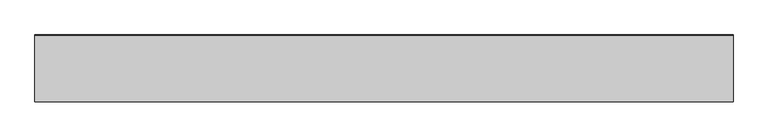
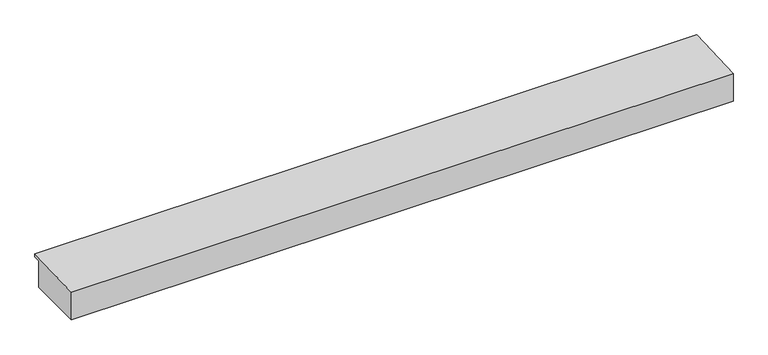
"""IFC4 building model written with IfcOpenShell, lengths in millimetres: proxy geometry, Generic Models 7:Generic Models 1:2:Generic Models 1:2 : Generic Models 7:Generic Models 1:337419:12 : Generic Models 7:Generic Models 1:2:Generic Models 1:2 : Generic Models 7:Generic Models 1:337419:306751."""

from ifc_helpers import new_model, si_unit, frame, origin, place, context, project, spatial, polyline, outline, extrude, source, transform, mapped, element, save


def generic_models_a1c6fa57(model_context):
    return source(origin(), model_context, "Body", "SweptSolid", [
        extrude(outline(polyline([(-578769.8021, 3730.7203868), (-578769.3002989, 3718.0302757), (-578794.3163841, 3716.9879388), (-578794.3163841, 3614.6261997), (-579001.9953617, 3614.6261997), (-579001.9953617, 3721.0456676), (-578769.8021, 3730.7203868)])), frame((591306.0367239, 0.0, 0.0), z_axis=(1.0, 0.0, 0.0), x_axis=(0.0, 1.0, 0.0)), (0.0, 0.0, 1.0), 2432.05),
    ])


if __name__ == "__main__":
    model = new_model("IFC4")
    model_context = context("Model", 3, world=origin())
    ifc_project = project(units=[si_unit("LENGTHUNIT", "METRE", prefix="MILLI")], contexts=[model_context])
    site = spatial("IfcSite", under=ifc_project)
    building = spatial("IfcBuilding", under=site)
    placement = place(None, origin())
    generic_models_shape = generic_models_a1c6fa57(model_context)
    element("IfcBuildingElementProxy", 1, Name="Generic Models 7:Generic Models 1:2:Generic Models 1:2 : Generic Models 7:Generic Models 1:337419:12 : Generic Models 7:Generic Models 1:2:Generic Models 1:2 : Generic Models 7:Generic Models 1:337419:306751", ObjectType="Generic Models 7:Generic Models 1:2:Generic Models 1:2 : Generic Models 7:Generic Models 1:337419:12 : Generic Models 7:Generic Models 1:2:Generic Models 1:2 : Generic Models 7:Generic Models 1:337419:306751", at=placement, inside=building, context=model_context, shape_type="MappedRepresentation", body=[
        mapped(generic_models_shape, transform((0.0, 0.0, 0.0), x_axis=(1.0, 0.0, 0.0), y_axis=(0.0, 1.0, 0.0), z_axis=(0.0, 0.0, 1.0))),
    ])
    save(model, "model.ifc")

# Revit data of these elements
# Type "Generic Models 7:Generic Models 1:2:Generic Models 1:2 : Generic Models 7:Generic Models 1:337419:12 : Generic Models 7:Generic Models 1:2:Generic Models 1:2 : Generic Models 7:Generic Models 1:337419:306751"
#   NameOverride = "Generic Models 7:Generic Models 1:2:Generic Models 1:2 : Generic Models 7:Generic Models 1:337419:306751"
#   ObjectTypeOverride = "Generic Models 1:2 : Generic Models 7:Generic Models 1:337419"
#   Reference = "Generic Models 1"
#   Tag = "306751"
# Element 1 (IfcBuildingElementProxy, "Generic Models 7:Generic Models 1:2:Generic Models 1:2 : Generic Models 7:Generic Models 1:337419:12 : Generic Models 7:Generic Models 1:2:Generic Models 1:2 : Generic Models 7:Generic Models 1:337419:306751")
#   Materials on its faces: "FULL CAVITY CLASS A FIBERGLASS INSULATION WITH DURABLE VAPOR BARRIER (BLACK) LINER"
# Materials
#   "FULL CAVITY CLASS A FIBERGLASS INSULATION WITH DURABLE VAPOR BARRIER (BLACK) LINER": class "Unassigned", colour RGB 158 92 175, transparency 0, Cost = 0
